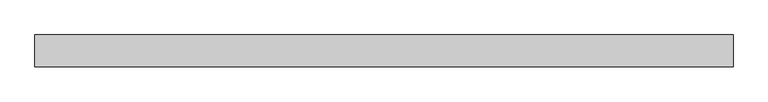
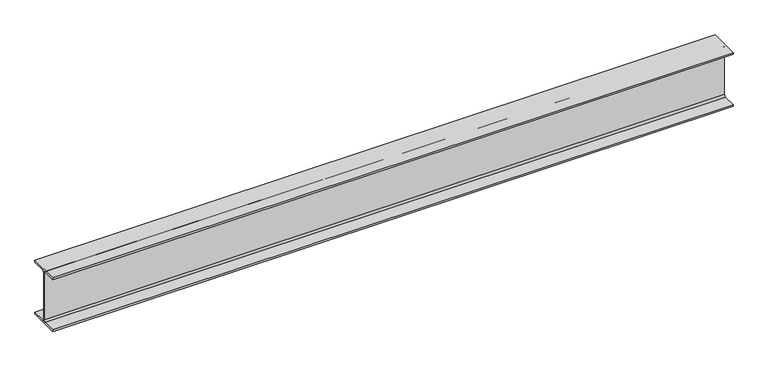
"""IFC4 building model written with IfcOpenShell, lengths in millimetres: beam geometry, Old_Steel Beam_H-KSD3502 : H_SB_ASB_H-200×200x8x12."""

from ifc_helpers import new_model, si_unit, point, frame, frame_2d, origin, place, context, project, spatial, polyline, circle_curve, trimmed, segment, composite_curve, outline, extrude, source, transform, mapped, element, save


def beam_d849abf2(model_context):
    return source(origin(), model_context, "Body", "SweptSolid", [
        extrude(outline(composite_curve([segment(polyline([(82.5, -141.5), (82.5, -151.7), (-82.5, -151.7), (-82.5, -141.5), (-11.9, -141.5)]), True, "CONTINUOUS"), segment(trimmed(circle_curve(frame_2d((-11.9, -132.6)), 8.9), [point((-11.9, -141.5))], [point((-3.0, -132.6))], True, "CARTESIAN"), True, "CONTINUOUS"), segment(polyline([(-3.0, -132.6), (-3.0, 132.6)]), True, "CONTINUOUS"), segment(trimmed(circle_curve(frame_2d((-11.9, 132.6)), 8.9), [point((-3.0, 132.6))], [point((-11.9, 141.5))], True, "CARTESIAN"), True, "CONTINUOUS"), segment(polyline([(-11.9, 141.5), (-82.5, 141.5), (-82.5, 151.7), (82.5, 151.7), (82.5, 141.5), (11.9, 141.5)]), True, "CONTINUOUS"), segment(trimmed(circle_curve(frame_2d((11.9, 132.6)), 8.9), [point((11.9, 141.5))], [point((3.0, 132.6))], True, "CARTESIAN"), True, "CONTINUOUS"), segment(polyline([(3.0, 132.6), (3.0, -132.6)]), True, "CONTINUOUS"), segment(trimmed(circle_curve(frame_2d((11.9, -132.6)), 8.9), [point((3.0, -132.6))], [point((11.9, -141.5))], True, "CARTESIAN"), True, "CONTINUOUS"), segment(polyline([(11.9, -141.5), (82.5, -141.5)]), True, "CONTINUOUS")], self_intersect=False)), frame((-1850.8543264, 0.0, 0.0), z_axis=(1.0, 0.0, 0.0), x_axis=(0.0, 1.0, 0.0)), (0.0, 0.0, 1.0), 3630.9979746),
    ])


if __name__ == "__main__":
    model = new_model("IFC4")
    model_context = context("Model", 3, world=origin())
    ifc_project = project(units=[si_unit("LENGTHUNIT", "METRE", prefix="MILLI")], contexts=[model_context])
    site = spatial("IfcSite", under=ifc_project)
    building = spatial("IfcBuilding", under=site)
    placement = place(None, origin())
    beam_shape = beam_d849abf2(model_context)
    element("IfcBeam", 1, ObjectType="Old_Steel Beam_H-KSD3502 : H_SB_ASB_H-200×200x8x12", at=placement, inside=building, context=model_context, shape_type="MappedRepresentation", body=[
        mapped(beam_shape, transform((0.0, 0.0, 0.0), x_axis=(1.0, 0.0, 0.0), y_axis=(0.0, 1.0, 0.0), z_axis=(0.0, 0.0, 1.0))),
    ])
    save(model, "model.ifc")

# Revit data of these elements
# Type "Old_Steel Beam_H-KSD3502 : H_SB_ASB_H-200×200x8x12"
#   Width = 20.0 cm
#   Web Thickness = 0.8 cm
#   Web Fillet = 1.3 cm
#   Warping Constant = 141376.0 cm⁶
#   Torsional Moment of Inertia = 26.2485 cm⁴
#   Torsional Modulus = 1.0 cm³
#   Section Area = 63.53 cm²
#   Plastic Modulus weak axis = 244.0 cm³
#   Plastic Modulus strong axis = 525.0 cm³
#   Perimeter = 1.16 m²/m
#   Nominal Weight = 49.90 kgf/m
#   Moment of Inertia weak axis = 1600.00 cm⁴
#   Moment of Inertia strong axis = 4720.00 cm⁴
#   Height = 20.0 cm
#   Flange Thickness = 1.2 cm
#   Elastic Modulus weak axis = 160.0 cm³
#   Elastic Modulus strong axis = 472.0 cm³
#   Centroid Vertical = 10.0 cm
#   Centroid Horizontal = 10.0 cm
#   Length [instance default] = 1.5240 m
#   Structural Material [instance default] = Steel, 45-345
#   Assembly Code = ""
# Element 1 (IfcBeam, "Old_Steel Beam_H-KSD3502 : H_SB_ASB_H-200×200x8x12")
#   Structural Material = none
# Materials
#   "Steel, 45-345": class "Metal", colour RGB 189 187 185, transparency 0, Description = "Steel 345 MPa", Cost = 0
